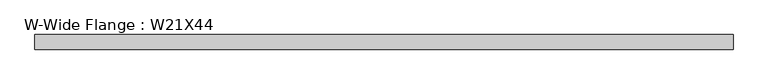
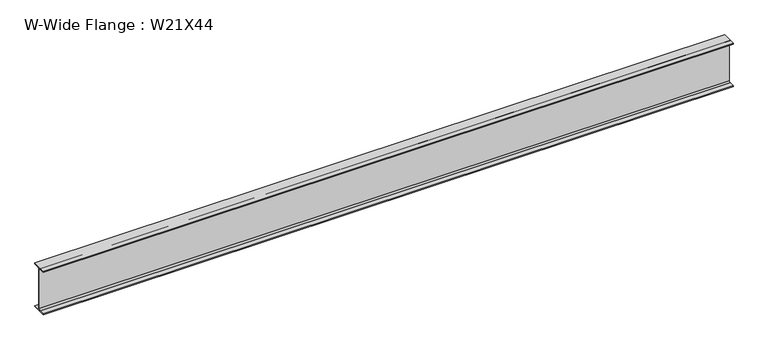
"""IFC4 building model written with IfcOpenShell, lengths in millimetres: beam geometry, W-Wide Flange : W21X44."""

from ifc_helpers import new_model, si_unit, point, frame, frame_2d, origin, place, context, project, spatial, polyline, circle_curve, trimmed, segment, composite_curve, outline, extrude, source, transform, mapped, element, save


def w_wide_flange_w21x44_bd7c8782(model_context):
    return source(origin(), model_context, "Body", "SweptSolid", [
        extrude(outline(composite_curve([segment(polyline([(82.55, -251.46), (82.55, -262.89), (-82.55, -262.89), (-82.55, -251.46), (-21.59, -251.46)]), True, "CONTINUOUS"), segment(trimmed(circle_curve(frame_2d((-21.59, -234.315)), 17.145), [point((-21.59, -251.46))], [point((-4.445, -234.315))], True, "CARTESIAN"), True, "CONTINUOUS"), segment(polyline([(-4.445, -234.315), (-4.445, 234.315)]), True, "CONTINUOUS"), segment(trimmed(circle_curve(frame_2d((-21.59, 234.315)), 17.145), [point((-4.445, 234.315))], [point((-21.59, 251.46))], True, "CARTESIAN"), True, "CONTINUOUS"), segment(polyline([(-21.59, 251.46), (-82.55, 251.46), (-82.55, 262.89), (82.55, 262.89), (82.55, 251.46), (21.59, 251.46)]), True, "CONTINUOUS"), segment(trimmed(circle_curve(frame_2d((21.59, 234.315)), 17.145), [point((21.59, 251.46))], [point((4.445, 234.315))], True, "CARTESIAN"), True, "CONTINUOUS"), segment(polyline([(4.445, 234.315), (4.445, -234.315)]), True, "CONTINUOUS"), segment(trimmed(circle_curve(frame_2d((21.59, -234.315)), 17.145), [point((4.445, -234.315))], [point((21.59, -251.46))], True, "CARTESIAN"), True, "CONTINUOUS"), segment(polyline([(21.59, -251.46), (82.55, -251.46)]), True, "CONTINUOUS")], self_intersect=False)), frame((-3902.7950665, 0.0, 0.0), z_axis=(1.0, 0.0, 0.0), x_axis=(0.0, 1.0, 0.0)), (0.0, 0.0, 1.0), 7866.2934453),
    ])


if __name__ == "__main__":
    model = new_model("IFC4")
    model_context = context("Model", 3, world=origin())
    ifc_project = project(units=[si_unit("LENGTHUNIT", "METRE", prefix="MILLI")], contexts=[model_context])
    site = spatial("IfcSite", under=ifc_project)
    building = spatial("IfcBuilding", under=site)
    placement = place(None, origin())
    w_wide_flange_w21x44_shape = w_wide_flange_w21x44_bd7c8782(model_context)
    element("IfcBeam", 1, ObjectType="W-Wide Flange : W21X44", at=placement, inside=building, context=model_context, shape_type="MappedRepresentation", body=[
        mapped(w_wide_flange_w21x44_shape, transform((0.0, 0.0, 0.0), x_axis=(1.0, 0.0, 0.0), y_axis=(0.0, 1.0, 0.0), z_axis=(0.0, 0.0, 1.0))),
    ])
    save(model, "model.ifc")

# Revit data of these elements
# Type "W-Wide Flange : W21X44"
#   Assembly Code = "B10"
#   W = 44
#   Length [instance default] = 1524 mm
#   bf = 165.1 mm
#   d = 525.78 mm
#   k = 28.575 mm
#   k2 = 17.145 mm
#   tf = 11.43 mm
#   tw = 8.89 mm
#   A = 0.00838708 m²
#   Structural Material [instance default] = Steel ASTM A992
# Element 1 (IfcBeam, "W-Wide Flange : W21X44")
#   Structural Material = Aluminum, Anodized Red
#   Materials on its faces: "Aluminum, Anodized Red"
# Materials
#   "Steel ASTM A992": class "Metal", colour RGB 128 0 0, transparency 0, Description = "Structural steel 50ksi", Cost = 0
#   "Aluminum, Anodized Red": class "Metal", colour RGB 120 120 120, transparency 0, Description = "Anodized aluminum, red", Cost = 0
